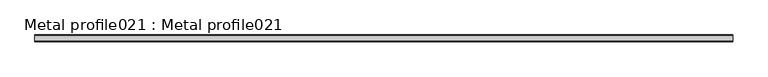
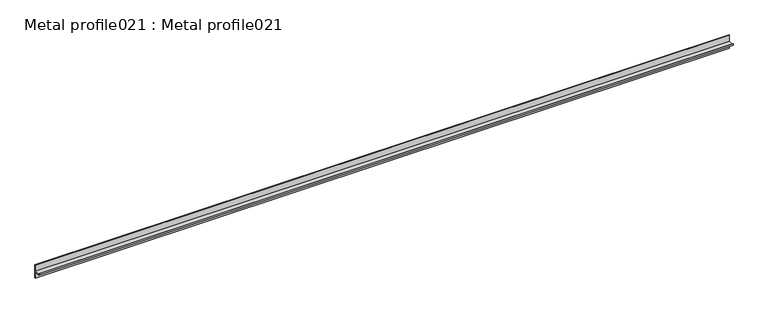
"""IFC4 building model written with IfcOpenShell, lengths in millimetres: proxy geometry, Metal profile021 : Metal profile021."""

from ifc_helpers import new_model, si_unit, frame, origin, place, context, project, spatial, polyline, outline, extrude, source, transform, mapped, element, save


def metal_profile021_metal_profile021_fe7b6f54(model_context):
    return source(origin(), model_context, "Body", "SweptSolid", [
        extrude(outline(polyline([(-4684.6182816, 39033.566875), (-4667.6543336, 39033.566875), (-4667.6543336, 39052.616875), (-4666.3843336, 39052.616875), (-4666.3843336, 39013.246875), (-4667.6543336, 39013.246875), (-4667.6543336, 39032.296875), (-4685.8882816, 39032.296875), (-4685.8882816, 39037.046675), (-4684.6182816, 39037.046675), (-4684.6182816, 39033.566875)])), frame((12383.0178845, 0.0, 0.0), z_axis=(1.0, 0.0, 0.0), x_axis=(0.0, 1.0, 0.0)), (0.0, 0.0, 1.0), 2000.0),
    ])


if __name__ == "__main__":
    model = new_model("IFC4")
    model_context = context("Model", 3, world=origin())
    ifc_project = project(units=[si_unit("LENGTHUNIT", "METRE", prefix="MILLI")], contexts=[model_context])
    site = spatial("IfcSite", under=ifc_project)
    building = spatial("IfcBuilding", under=site)
    placement = place(None, origin())
    metal_profile021_metal_profile021_shape = metal_profile021_metal_profile021_fe7b6f54(model_context)
    element("IfcBuildingElementProxy", 1, Name="Metal profile021 : Metal profile021", ObjectType="Metal profile021 : Metal profile021", at=placement, inside=building, context=model_context, shape_type="MappedRepresentation", body=[
        mapped(metal_profile021_metal_profile021_shape, transform((0.0, 0.0, 0.0), x_axis=(1.0, 0.0, 0.0), y_axis=(0.0, 1.0, 0.0), z_axis=(0.0, 0.0, 1.0))),
    ])
    save(model, "model.ifc")

# Revit data of these elements
# Type "Metal profile021 : Metal profile021"
#   NameOverride = "Metal profile021"
# Element 1 (IfcBuildingElementProxy, "Metal profile021 : Metal profile021")
#   Materials on its faces: "16 GA. COPPER VENTED T REVEAL BEAD"
# Materials
#   "16 GA. COPPER VENTED T REVEAL BEAD": class "Unassigned", colour RGB 255 227 10, transparency 0
